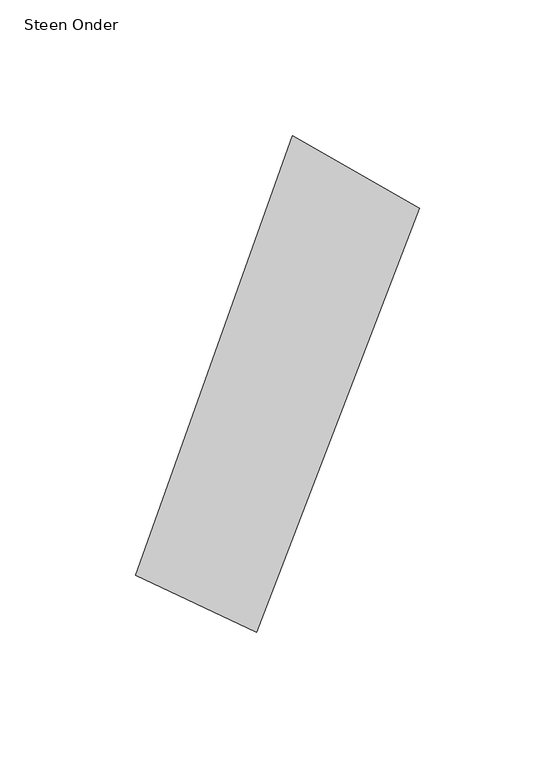
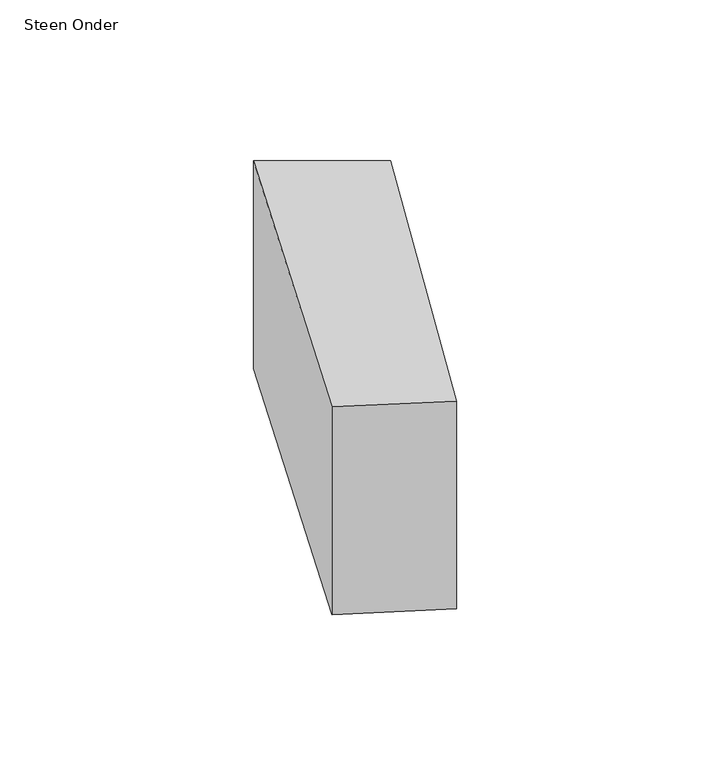
"""IFC4 building model written with IfcOpenShell, lengths in millimetres: proxy geometry, 00_GMA_steen_versie_4 : Steen Onder."""

import ifcopenshell
import ifcopenshell.guid

model = None  # the IFC model being written
_history = None  # IfcOwnerHistory: only IFC2X3 demands one
_inside = {}  # id of a spatial element -> (the spatial element, [elements in it])
_under = {}  # id of a project, library or spatial element -> (it, [spatial elements below it])
_declared = {}  # id of a project -> (the project, [libraries it declares])
_typed = {}  # id of a type object -> (the type object, [elements of that type])
_made_of = {}  # id of a material, layer set ... -> (it, [elements and type objects made of it])


def new_model(schema):
    """Start an empty IFC model of exactly this schema.

    Asked for "IFC4X3", IfcOpenShell would pick the latest addendum, in which some entities
    have other attributes; the version numbers below select the first issue.
    IFC2X3 requires an IfcOwnerHistory on every rooted entity: one is made here for all.
    """
    global model, _history
    if schema == "IFC4X3":
        model = ifcopenshell.file(schema_version=(4, 3, 0, 0))
    else:
        model = ifcopenshell.file(schema=schema)
    _inside.clear()
    _under.clear()
    _declared.clear()
    _typed.clear()
    _made_of.clear()
    _history = None
    if model.schema == "IFC2X3":
        org = make("IfcOrganization", Name="unknown")
        user = make(
            "IfcPersonAndOrganization",
            ThePerson=make("IfcPerson", FamilyName="unknown"),
            TheOrganization=org,
        )
        app = make(
            "IfcApplication",
            ApplicationDeveloper=org,
            Version="unknown",
            ApplicationFullName="unknown",
            ApplicationIdentifier="unknown",
        )
        _history = make(
            "IfcOwnerHistory",
            OwningUser=user,
            OwningApplication=app,
            ChangeAction="ADDED",
            CreationDate=0,
        )
    return model


def make(cls, **values):
    """One entity of the class cls with the attributes given. An attribute that is None is left unset."""
    return model.create_entity(
        cls, **{name: value for name, value in values.items() if value is not None}
    )


def rooted(cls, **values):
    """An entity with a GlobalId (a new one), such as an element, a storey or a relation."""
    return make(cls, GlobalId=ifcopenshell.guid.new(), OwnerHistory=_history, **values)


def si_unit(unit_type, name, prefix=None):
    """IfcSIUnit, for example si_unit("LENGTHUNIT", "METRE", prefix="MILLI")."""
    return make("IfcSIUnit", UnitType=unit_type, Prefix=prefix, Name=name)


def assignment(units):
    """IfcUnitAssignment: the units of a project."""
    return None if units is None else make("IfcUnitAssignment", Units=units)


def point(xyz):
    """IfcCartesianPoint."""
    return None if xyz is None else make("IfcCartesianPoint", Coordinates=xyz)


def direction(xyz):
    """IfcDirection."""
    return None if xyz is None else make("IfcDirection", DirectionRatios=xyz)


def frame(location, z_axis=None, x_axis=None):
    """IfcAxis2Placement3D, a coordinate frame: its origin and axes. An axis left out is left unset."""
    return make(
        "IfcAxis2Placement3D",
        Location=point(location),
        Axis=direction(z_axis),
        RefDirection=direction(x_axis),
    )


def origin():
    """The frame at (0, 0, 0) with its axes left unset."""
    return frame((0.0, 0.0, 0.0))


def origin_with_axes():
    """The frame at (0, 0, 0) with the z axis (0, 0, 1) and the x axis (1, 0, 0) written out."""
    return frame((0.0, 0.0, 0.0), z_axis=(0.0, 0.0, 1.0), x_axis=(1.0, 0.0, 0.0))


def place(relative_to, where):
    """IfcLocalPlacement: puts the frame where relative to a parent placement (None: the world)."""
    return make(
        "IfcLocalPlacement", PlacementRelTo=relative_to, RelativePlacement=where
    )


def context(
    kind, dimensions, precision=None, world=None, true_north=None, identifier=None
):
    """IfcGeometricRepresentationContext, for example the 3D "Model" context."""
    return make(
        "IfcGeometricRepresentationContext",
        ContextIdentifier=identifier,
        ContextType=kind,
        CoordinateSpaceDimension=dimensions,
        Precision=precision,
        WorldCoordinateSystem=world,
        TrueNorth=true_north,
    )


def project(units=None, contexts=None):
    """IfcProject with its units and contexts."""
    return rooted(
        "IfcProject",
        Name="project",
        RepresentationContexts=contexts,
        UnitsInContext=assignment(units),
    )


def spatial(cls, under=None, at=None, **own):
    """A site, building, storey or space (cls), placed at a placement, below another one or the project."""
    s = rooted(cls, ObjectPlacement=at, **own)
    if under is not None:
        _under.setdefault(under.id(), (under, []))[1].append(s)
    return s


def polyline(points):
    """IfcPolyline through the points."""
    return make("IfcPolyline", Points=[point(p) for p in points])


def outline(outer, holes=None, kind="AREA"):
    """IfcArbitraryClosedProfileDef: a profile drawn as a closed curve; with holes, ...WithVoids."""
    if holes is None:
        return make("IfcArbitraryClosedProfileDef", ProfileType=kind, OuterCurve=outer)
    return make(
        "IfcArbitraryProfileDefWithVoids",
        ProfileType=kind,
        OuterCurve=outer,
        InnerCurves=holes,
    )


def extrude(swept, where, along, depth):
    """IfcExtrudedAreaSolid: the profile swept, set in the frame where, extruded along a direction by depth."""
    return make(
        "IfcExtrudedAreaSolid",
        SweptArea=swept,
        Position=where,
        ExtrudedDirection=direction(along),
        Depth=depth,
    )


def shape(context_of_items, identifier, shape_type, items):
    """IfcShapeRepresentation: the items that make up one representation, for example the "Body"."""
    return make(
        "IfcShapeRepresentation",
        ContextOfItems=context_of_items,
        RepresentationIdentifier=identifier,
        RepresentationType=shape_type,
        Items=items,
    )


def source(mapping_origin, context_of_items, identifier, shape_type, items):
    """IfcRepresentationMap: a shape defined once, which mapped items show again and again."""
    return make(
        "IfcRepresentationMap",
        MappingOrigin=mapping_origin,
        MappedRepresentation=shape(context_of_items, identifier, shape_type, items),
    )


def transform(
    local_origin,
    x_axis=None,
    y_axis=None,
    z_axis=None,
    scale=None,
    scale2=None,
    scale3=None,
    uniform=True,
):
    """IfcCartesianTransformationOperator3D, or its non-uniform kind. x_axis, y_axis, z_axis: its Axis1, 2, 3."""
    if uniform:
        return make(
            "IfcCartesianTransformationOperator3D",
            Axis1=direction(x_axis),
            Axis2=direction(y_axis),
            LocalOrigin=point(local_origin),
            Scale=scale,
            Axis3=direction(z_axis),
        )
    return make(
        "IfcCartesianTransformationOperator3DnonUniform",
        Axis1=direction(x_axis),
        Axis2=direction(y_axis),
        LocalOrigin=point(local_origin),
        Scale=scale,
        Axis3=direction(z_axis),
        Scale2=scale2,
        Scale3=scale3,
    )


def mapped(mapping_source, mapping_target):
    """IfcMappedItem: shows the shape of a source again, moved by a transform."""
    return make(
        "IfcMappedItem", MappingSource=mapping_source, MappingTarget=mapping_target
    )


def made_of(thing, what):
    """Note that an element or type object is made of a material, layer set ...; save() writes the relation."""
    if what is not None:
        _made_of.setdefault(what.id(), (what, []))[1].append(thing)
    return thing


def element(
    cls,
    number,
    at=None,
    inside=None,
    cuts=None,
    type_object=None,
    material=None,
    context=None,
    identifier="Body",
    shape_type=None,
    held_by="IfcProductDefinitionShape",
    body=None,
    shapes=None,
    **own,
):
    """One element of the class cls, such as IfcWall. Its Tag is "e" and its number.

    at: its placement. inside: the storey or other place that contains it. cuts: it is an
    opening in that element (IfcRelVoidsElement). A single representation is given by context,
    identifier, shape_type and body (its items); several are given by shapes. held_by: the class
    of the entity that holds the representations. save() writes the other relations.
    """
    e = rooted(cls, Tag="e%d" % number, ObjectPlacement=at, **own)
    if body is not None:
        shapes = [shape(context, identifier, shape_type, body)]
    if shapes is not None:
        e.Representation = make(held_by, Representations=shapes)
    if inside is not None:
        _inside.setdefault(inside.id(), (inside, []))[1].append(e)
    if cuts is not None:
        rooted(
            "IfcRelVoidsElement", RelatingBuildingElement=cuts, RelatedOpeningElement=e
        )
    if type_object is not None:
        _typed.setdefault(type_object.id(), (type_object, []))[1].append(e)
    return made_of(e, material)


def aggregate(whole, parts):
    """IfcRelAggregates: a whole, such as a stair, and the parts it consists of."""
    return rooted("IfcRelAggregates", RelatingObject=whole, RelatedObjects=parts)


def save(model, path):
    """Write the relations noted so far, then the file.

    IfcRelAggregates (storeys below a building ...), IfcRelContainedInSpatialStructure (elements
    in a storey), IfcRelDefinesByType, IfcRelAssociatesMaterial and IfcRelDeclares: one each for
    every whole, place, type object, material and project.
    """
    for whole, parts in _under.values():
        aggregate(whole, parts)
    for where, things in _inside.values():
        rooted(
            "IfcRelContainedInSpatialStructure",
            RelatedElements=things,
            RelatingStructure=where,
        )
    for kind, things in _typed.values():
        rooted("IfcRelDefinesByType", RelatedObjects=things, RelatingType=kind)
    for what, things in _made_of.values():
        rooted("IfcRelAssociatesMaterial", RelatedObjects=things, RelatingMaterial=what)
    for by, libraries in _declared.values():
        rooted("IfcRelDeclares", RelatingContext=by, RelatedDefinitions=libraries)
    model.write(path)


def steen_onder_44ca1660(model_context):
    return source(origin(), model_context, "Body", "SweptSolid", [
        extrude(outline(polyline([(130.296874, 146.7969185), (70.2672261, -9.4223747), (25.6917369, 11.6233535), (83.5239747, 173.5535051), (130.296874, 146.7969185)])), origin_with_axes(), (0.0, 0.0, 1.0), 100.0),
    ])


if __name__ == "__main__":
    model = new_model("IFC4")
    model_context = context("Model", 3, world=origin())
    ifc_project = project(units=[si_unit("LENGTHUNIT", "METRE", prefix="MILLI")], contexts=[model_context])
    site = spatial("IfcSite", under=ifc_project)
    building = spatial("IfcBuilding", under=site)
    placement = place(None, origin())
    steen_onder_shape = steen_onder_44ca1660(model_context)
    element("IfcBuildingElementProxy", 1, Name="00_GMA_steen_versie_4 : Steen Onder", ObjectType="00_GMA_steen_versie_4 : Steen Onder", at=placement, inside=building, context=model_context, shape_type="MappedRepresentation", body=[
        mapped(steen_onder_shape, transform((0.0, 0.0, 0.0), x_axis=(1.0, 0.0, 0.0), y_axis=(0.0, 1.0, 0.0), z_axis=(0.0, 0.0, 1.0))),
    ])
    save(model, "model.ifc")

# Revit data of these elements
# Type "00_GMA_steen_versie_4 : Steen Onder"
#   StootVoegHalfBoven [instance default] = 5 mm
#   StootVoegHalf [instance default] = 5 mm
#   StootVoegBreedteOnder = 10 mm
#   StootVoegBreedteBoven = 10 mm
#   Steendikte = 100 mm
#   LintVoegOnderHalf = 0 mm
#   LintVoegOnder = 0 mm
#   LintVoegBovenHalf = 5 mm
#   LintVoegBoven = 10 mm
#   materiaal = none
#   MateriaalVoeg = none
#   Default Elevation = 0
